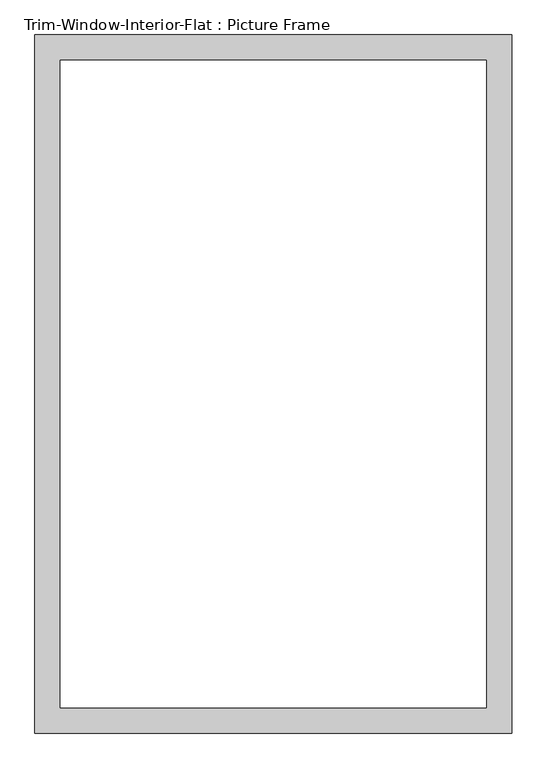
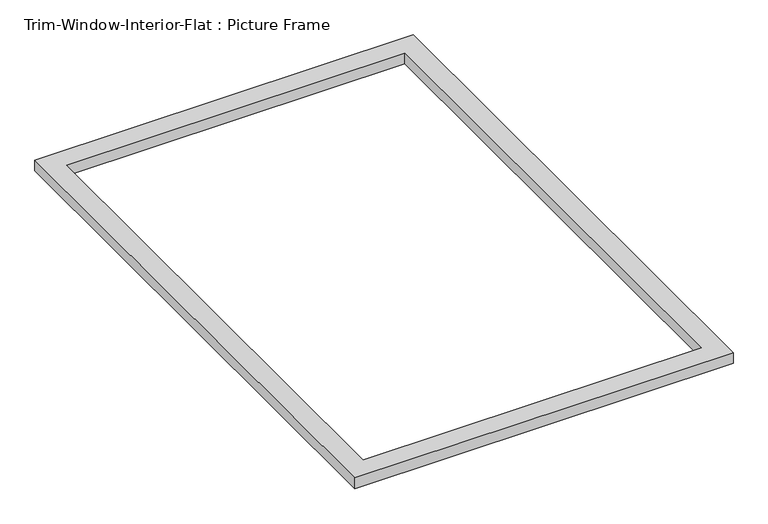
"""IFC4 building model written with IfcOpenShell, lengths in millimetres: proxy geometry, Trim-Window-Interior-Flat : Picture Frame."""

from ifc_helpers import new_model, si_unit, origin, origin_with_axes, place, context, project, spatial, polyline, outline, extrude, source, transform, mapped, element, save


def trim_window_interior_flat_picture_frame_52ad8ec8(model_context):
    return source(origin(), model_context, "Body", "SweptSolid", [
        extrude(outline(polyline([(533.4, -44.45), (-533.4, -44.45), (-533.4, 1517.65), (533.4, 1517.65), (533.4, -44.45)]), holes=[polyline([(476.25, 12.7), (476.25, 1460.5), (-476.25, 1460.5), (-476.25, 12.7), (476.25, 12.7)])]), origin_with_axes(), (0.0, 0.0, 1.0), 31.75),
    ])


if __name__ == "__main__":
    model = new_model("IFC4")
    model_context = context("Model", 3, world=origin())
    ifc_project = project(units=[si_unit("LENGTHUNIT", "METRE", prefix="MILLI")], contexts=[model_context])
    site = spatial("IfcSite", under=ifc_project)
    building = spatial("IfcBuilding", under=site)
    placement = place(None, origin())
    trim_window_interior_flat_picture_frame_shape = trim_window_interior_flat_picture_frame_52ad8ec8(model_context)
    element("IfcBuildingElementProxy", 1, Name="Trim-Window-Interior-Flat : Picture Frame", ObjectType="Trim-Window-Interior-Flat : Picture Frame", at=placement, inside=building, context=model_context, shape_type="MappedRepresentation", body=[
        mapped(trim_window_interior_flat_picture_frame_shape, transform((0.0, 0.0, 0.0), x_axis=(1.0, 0.0, 0.0), y_axis=(0.0, 1.0, 0.0), z_axis=(0.0, 0.0, 1.0))),
    ])
    save(model, "model.ifc")

# Revit data of these elements
# Type "Trim-Window-Interior-Flat : Picture Frame"
#   Trim Thickness_Picture Frame = 0' - 1 1/4"
#   Trim Width = 0' - 2 1/4"
#   Trim Thickness_with Sill = 0' - 0 3/4"
#   Sill Thickness = 0' - 1 1/4"
#   Opening Width [instance default] = 2' - 0"
#   Opening Height [instance default] = 3' - 0"
#   Default Elevation = 4' - 0"
#   Sill = no
#   Picture Frame = yes
#   Trim Material [instance default] = none
# Element 1 (IfcBuildingElementProxy, "Trim-Window-Interior-Flat : Picture Frame")
#   Opening Width = 3' - 2 1/2"
#   Opening Height = 4' - 10"
#   Trim Material = Wood - Stained
#   Materials on its faces: "Wood - Stained"
# Materials
#   "Wood - Stained": class "Wood", colour RGB 224 178 126, transparency 0, Cost = 0
